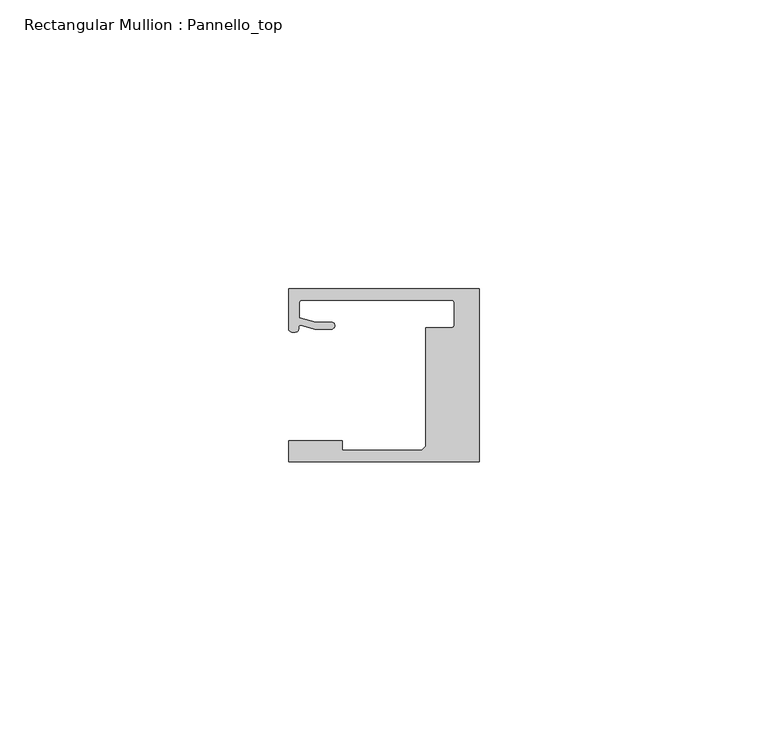
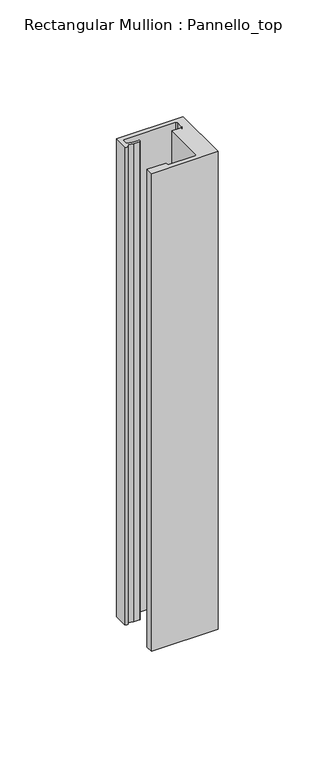
"""IFC4 building model written with IfcOpenShell, lengths in millimetres: member geometry, Rectangular Mullion : Pannello_top."""

from ifc_helpers import new_model, si_unit, frame, origin, place, context, project, spatial, polyline, circle_curve, source, transform, mapped, element, save
from ifc_brep_helpers import plane_surface, cylinder_surface, revolved_surface, extruded_surface, spline_curve, advanced_brep


def rectangular_mullion_pannello_top_1a123040(model_context):
    return source(origin(), model_context, "Body", "AdvancedBrep", [
        advanced_brep(
        [(-33.0, -15.0, 0.0), (0.0, -15.0, 0.0), (0.0, 15.0, 0.0), (-33.0000135, 15.0, 0.0), (-33.0000135, 8.0000472, 0.0), (-30.9223017, 8.6490241, 0.0), (-28.4999305, 7.9999523, 0.0), (-25.59998, 7.9999523, 0.0), (-25.59998, 9.1999523, 0.0), (-28.3419477, 9.1999523, 0.0), (-31.19998, 9.9657591, 0.0), (-31.19998, 12.50001, 0.0), (-30.69998, 13.00001, 0.0), (-4.7999726, 13.00001, 0.0), (-4.2999726, 12.50001, 0.0), (-4.2999726, 8.7500595, 0.0), (-4.7999726, 8.2500595, 0.0), (-9.2999726, 8.2500595, 0.0), (-9.2999726, -12.2999849, 0.0), (-10.0000103, -13.0000004, 0.0), (-23.700041, -13.0000004, 0.0), (-23.700041, -11.3000004, 0.0), (-33.0, -11.3000004, 0.0), (-33.0, -15.0, -250.0), (-33.0, -11.3000004, -250.0), (-23.700041, -11.3000004, -250.0), (-23.700041, -13.0000004, -250.0), (-10.0000103, -13.0000004, -250.0), (-9.2999726, -12.2999849, -250.0), (-9.2999726, 8.2500595, -250.0), (-4.7999726, 8.2500595, -250.0), (-4.2999726, 8.7500595, -250.0), (-4.2999726, 12.50001, -250.0), (-4.7999726, 13.00001, -250.0), (-30.69998, 13.00001, -250.0), (-31.19998, 12.50001, -250.0), (-31.19998, 9.9657591, -250.0), (-28.3419477, 9.1999523, -250.0), (-25.59998, 9.1999523, -250.0), (-25.59998, 7.9999523, -250.0), (-28.4999305, 7.9999523, -250.0), (-30.9223017, 8.6490241, -250.0), (-33.0000135, 8.0000472, -250.0), (-33.0000135, 15.0, -250.0), (0.0, 15.0, -250.0), (0.0, -15.0, -250.0)],
        [
            (0, 1),
            (1, 2),
            (2, 3),
            (3, 4),
            (4, 5, spline_curve(3, [(-33.0000135, 8.0000472, 0.0), (-33.0000135, 7.457047519, 0.0), (-32.262327879, 7.456527435, 0.0), (-31.357433266, 7.563996614, 0.0), (-31.305645054, 7.690065204, 0.0), (-31.298563602, 8.366228555, 0.0), (-31.312054066, 8.717747958, 0.0), (-30.9223017, 8.6490241, 0.0)], [4, 2, 2, 4], [0.0, 0.0027053965905959043, 0.0058611956533709, 0.007702013405570312])),
            (5, 6),
            (6, 7),
            (7, 8, circle_curve(frame((-25.59998, 8.5999523, 0.0), z_axis=(0.0, 0.0, 1.0), x_axis=(0.0, 1.0, 0.0)), 0.6)),
            (8, 9),
            (9, 10),
            (10, 11),
            (11, 12, circle_curve(frame((-30.69998, 12.50001, 0.0), z_axis=(0.0, 0.0, -1.0), x_axis=(0.0, 1.0, 0.0)), 0.5)),
            (12, 13),
            (13, 14, circle_curve(frame((-4.7999726, 12.50001, 0.0), z_axis=(0.0, 0.0, -1.0), x_axis=(1.0, 0.0, 0.0)), 0.5)),
            (14, 15),
            (15, 16, circle_curve(frame((-4.7999726, 8.7500595, 0.0), z_axis=(0.0, 0.0, -1.0), x_axis=(0.0, -1.0, 0.0)), 0.5)),
            (16, 17),
            (17, 18),
            (18, 19),
            (19, 20),
            (20, 21),
            (21, 22),
            (22, 0),
            (23, 24),
            (24, 25),
            (25, 26),
            (26, 27),
            (27, 28),
            (28, 29),
            (29, 30),
            (30, 31, circle_curve(frame((-4.7999726, 8.7500595, -250.0), z_axis=(0.0, 0.0, 1.0), x_axis=(0.0, -1.0, 0.0)), 0.5)),
            (31, 32),
            (32, 33, circle_curve(frame((-4.7999726, 12.50001, -250.0), z_axis=(0.0, 0.0, 1.0), x_axis=(1.0, 0.0, 0.0)), 0.5)),
            (33, 34),
            (34, 35, circle_curve(frame((-30.69998, 12.50001, -250.0), z_axis=(0.0, 0.0, 1.0), x_axis=(0.0, 1.0, 0.0)), 0.5)),
            (35, 36),
            (36, 37),
            (37, 38),
            (38, 39, circle_curve(frame((-25.59998, 8.5999523, -250.0), z_axis=(0.0, 0.0, -1.0), x_axis=(0.0, 1.0, 0.0)), 0.6)),
            (39, 40),
            (40, 41),
            (41, 42, spline_curve(3, [(-30.9223017, 8.6490241, -250.0), (-31.312054066, 8.717747958, -250.0), (-31.298563602, 8.366228555, -250.0), (-31.305645054, 7.690065204, -250.0), (-31.357433266, 7.563996614, -250.0), (-32.262327879, 7.456527435, -250.0), (-33.0000135, 7.457047519, -250.0), (-33.0000135, 8.0000472, -250.0)], [4, 2, 2, 4], [0.0, 0.001840817752199412, 0.004996616814974408, 0.007702013405570312])),
            (42, 43),
            (43, 44),
            (44, 45),
            (45, 23),
            (0, 23),
            (45, 1),
            (44, 2),
            (43, 3),
            (42, 4),
            (41, 5),
            (40, 6),
            (39, 7),
            (38, 8),
            (37, 9),
            (36, 10),
            (35, 11),
            (34, 12),
            (33, 13),
            (32, 14),
            (31, 15),
            (30, 16),
            (29, 17),
            (28, 18),
            (27, 19),
            (26, 20),
            (25, 21),
            (24, 22),
        ],
        [
            plane_surface(frame((0.0, -36.2491502, 0.0), z_axis=(0.0, 0.0, 1.0), x_axis=(-1.0, 0.0, 0.0))),
            plane_surface(frame((0.0, -36.2491502, -250.0), z_axis=(0.0, 0.0, -1.0), x_axis=(-1.0, 0.0, 0.0))),
            plane_surface(frame((-33.0, -15.0, 0.0), z_axis=(0.0, -1.0, 0.0), x_axis=(0.0, 0.0, -1.0))),
            plane_surface(frame((0.0, -15.0, 0.0), z_axis=(1.0, 0.0, 0.0), x_axis=(0.0, 0.0, -1.0))),
            plane_surface(frame((0.0, 15.0, 0.0), z_axis=(0.0, 1.0, 0.0), x_axis=(0.0, 0.0, -1.0))),
            plane_surface(frame((-33.0000135, 15.0, 0.0), z_axis=(-1.0, 0.0, 0.0), x_axis=(0.0, 0.0, -1.0))),
            extruded_surface(spline_curve(3, [(-33.0000135, 8.0000472, -250.0), (-33.0000135, 7.457047519, -250.0), (-32.262327879, 7.456527435, -250.0), (-31.357433266, 7.563996614, -250.0), (-31.305645054, 7.690065204, -250.0), (-31.298563602, 8.366228555, -250.0), (-31.312054066, 8.717747958, -250.0), (-30.9223017, 8.6490241, -250.0)], [4, 2, 2, 4], [0.0, 0.0027053965905959043, 0.0058611956533709, 0.007702013405570312]), (0.0, 0.0, 250.0), 250.0),
            plane_surface(frame((-30.9223017, 8.6490241, 0.0), z_axis=(-0.25881883200192934, -0.9659258833891746, 0.0), x_axis=(0.0, 0.0, -1.0))),
            plane_surface(frame((-28.4999305, 7.9999523, 0.0), z_axis=(0.0, -1.0, 0.0), x_axis=(0.0, 0.0, -1.0))),
            cylinder_surface(frame((-25.59998, 8.5999523, 0.0), z_axis=(0.0, 0.0, 1.0), x_axis=(0.0, 1.0, 0.0)), 0.6),
            plane_surface(frame((-25.59998, 9.1999523, 0.0), z_axis=(0.0, 1.0, 0.0), x_axis=(0.0, 0.0, -1.0))),
            plane_surface(frame((-28.3419477, 9.1999523, 0.0), z_axis=(0.25881883204288636, 0.9659258833782002, 0.0), x_axis=(0.0, 0.0, -1.0))),
            plane_surface(frame((-31.19998, 9.9657591, 0.0), z_axis=(1.0, 0.0, 0.0), x_axis=(0.0, 0.0, -1.0))),
            revolved_surface(polyline([(-30.69998, 13.00001, -250.0), (-30.69998, 13.00001, 0.0)]), (-30.69998, 12.50001, 0.0), (0.0, 0.0, -1.0)),
            plane_surface(frame((-30.69998, 13.00001, 0.0), z_axis=(0.0, -1.0, 0.0), x_axis=(0.0, 0.0, -1.0))),
            revolved_surface(polyline([(-4.2999726, 12.50001, -250.0), (-4.2999726, 12.50001, 0.0)]), (-4.7999726, 12.50001, 0.0), (0.0, 0.0, -1.0)),
            plane_surface(frame((-4.2999726, 12.50001, 0.0), z_axis=(-1.0, 0.0, 0.0), x_axis=(0.0, 0.0, -1.0))),
            revolved_surface(polyline([(-4.7999726, 8.2500595, -250.0), (-4.7999726, 8.2500595, 0.0)]), (-4.7999726, 8.7500595, 0.0), (0.0, 0.0, -1.0)),
            plane_surface(frame((-4.7999726, 8.2500595, 0.0), z_axis=(0.0, 1.0, 0.0), x_axis=(0.0, 0.0, -1.0))),
            plane_surface(frame((-9.2999726, 8.2500595, 0.0), z_axis=(-1.0, 0.0, 0.0), x_axis=(0.0, 0.0, -1.0))),
            plane_surface(frame((-9.2999726, -12.2999849, 0.0), z_axis=(-0.7070955486277984, 0.7071180135668678, 0.0), x_axis=(0.0, 0.0, -1.0))),
            plane_surface(frame((-10.0000103, -13.0000004, 0.0), z_axis=(0.0, 1.0, 0.0), x_axis=(0.0, 0.0, -1.0))),
            plane_surface(frame((-23.700041, -13.0000004, 0.0), z_axis=(1.0, 0.0, 0.0), x_axis=(0.0, 0.0, -1.0))),
            plane_surface(frame((-23.700041, -11.3000004, 0.0), z_axis=(0.0, 1.0, 0.0), x_axis=(0.0, 0.0, -1.0))),
            plane_surface(frame((-33.0, -11.3000004, 0.0), z_axis=(-1.0, 0.0, 0.0), x_axis=(0.0, 0.0, -1.0))),
        ],
        [
            (0, [[1, 2, 3, 4, 5, 6, 7, 8, 9, 10, 11, 12, 13, 14, 15, 16, 17, 18, 19, 20, 21, 22, 23]]),
            (1, [[24, 25, 26, 27, 28, 29, 30, 31, 32, 33, 34, 35, 36, 37, 38, 39, 40, 41, 42, 43, 44, 45, 46]]),
            (2, [[-1, 47, -46, 48]]),
            (3, [[-2, -48, -45, 49]]),
            (4, [[-3, -49, -44, 50]]),
            (5, [[-4, -50, -43, 51]]),
            (6, [[-5, -51, -42, 52]]),
            (7, [[-6, -52, -41, 53]]),
            (8, [[-7, -53, -40, 54]]),
            (9, [[-8, -54, -39, 55]]),
            (10, [[-9, -55, -38, 56]]),
            (11, [[-10, -56, -37, 57]]),
            (12, [[-11, -57, -36, 58]]),
            (13, [[-12, -58, -35, 59]]),
            (14, [[-13, -59, -34, 60]]),
            (15, [[-14, -60, -33, 61]]),
            (16, [[-15, -61, -32, 62]]),
            (17, [[-16, -62, -31, 63]]),
            (18, [[-17, -63, -30, 64]]),
            (19, [[-18, -64, -29, 65]]),
            (20, [[-19, -65, -28, 66]]),
            (21, [[-20, -66, -27, 67]]),
            (22, [[-21, -67, -26, 68]]),
            (23, [[-22, -68, -25, 69]]),
            (24, [[-23, -69, -24, -47]]),
        ],
    ),
    ])


if __name__ == "__main__":
    model = new_model("IFC4")
    model_context = context("Model", 3, world=origin())
    ifc_project = project(units=[si_unit("LENGTHUNIT", "METRE", prefix="MILLI")], contexts=[model_context])
    site = spatial("IfcSite", under=ifc_project)
    building = spatial("IfcBuilding", under=site)
    placement = place(None, origin())
    rectangular_mullion_pannello_top_shape = rectangular_mullion_pannello_top_1a123040(model_context)
    element("IfcMember", 1, ObjectType="Rectangular Mullion : Pannello_top", at=placement, inside=building, context=model_context, shape_type="MappedRepresentation", body=[
        mapped(rectangular_mullion_pannello_top_shape, transform((0.0, 0.0, 0.0), x_axis=(1.0, 0.0, 0.0), y_axis=(0.0, 1.0, 0.0), z_axis=(0.0, 0.0, 1.0))),
    ])
    save(model, "model.ifc")

# Revit data of these elements
# Type "Rectangular Mullion : Pannello_top"
#   built-in parameter 1007322 = 0.0984252 (stored number, unit not read)
#   built-in parameter 1007321 = 0 (stored number, unit not read)
#   built-in parameter 1007320 = 0.0305117 (stored number, unit not read)
